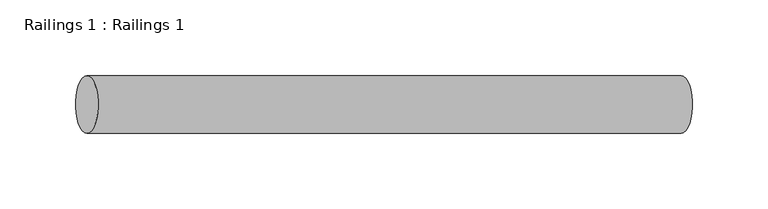
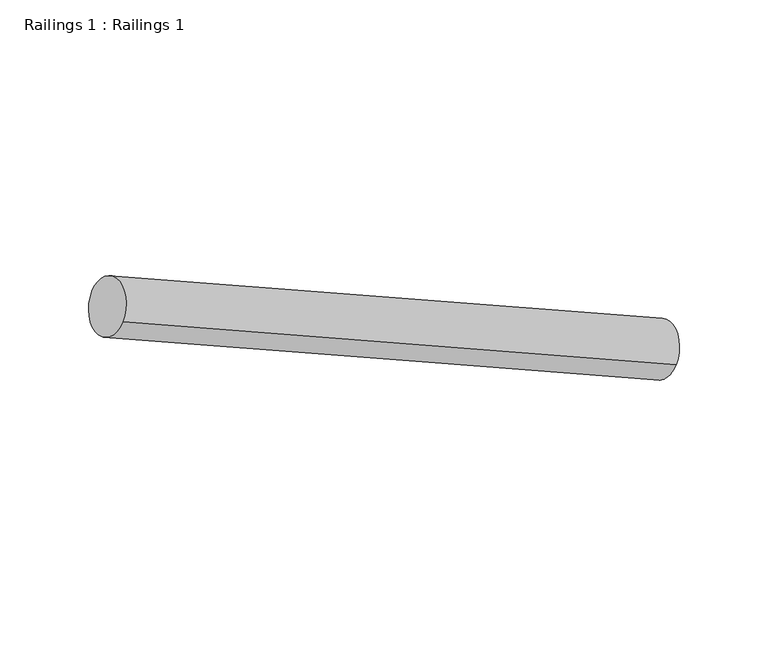
"""IFC4 building model written with IfcOpenShell, lengths in millimetres: railing geometry, Railings 1 : Railings 1."""

from ifc_helpers import new_model, si_unit, point, frame, frame_2d, origin, place, context, project, spatial, circle_curve, trimmed, segment, composite_curve, outline, extrude, source, transform, mapped, element, save


def railings_1_railings_1_71f28f68(model_context):
    return source(origin(), model_context, "Body", "SweptSolid", [
        extrude(outline(composite_curve([segment(trimmed(circle_curve(frame_2d((0.0, -19.05)), 19.05), [point((0.0, -38.1))], [point((0.0, 0.0))], False, "CARTESIAN"), True, "CONTINUOUS"), segment(trimmed(circle_curve(frame_2d((0.0, -19.05)), 19.05), [point((0.0, 0.0))], [point((0.0, -38.1))], False, "CARTESIAN"), True, "CONTINUOUS")], self_intersect=False)), frame((27413.4762341, 3829.6727004, 2323.0746661), z_axis=(-0.9180751215985248, 0.0, 0.39640644684698806), x_axis=(-0.39640644684698806, 0.0, -0.9180751215985248)), (0.0, 0.0, 1.0), 428.2410903),
    ])


if __name__ == "__main__":
    model = new_model("IFC4")
    model_context = context("Model", 3, world=origin())
    ifc_project = project(units=[si_unit("LENGTHUNIT", "METRE", prefix="MILLI")], contexts=[model_context])
    site = spatial("IfcSite", under=ifc_project)
    building = spatial("IfcBuilding", under=site)
    placement = place(None, origin())
    railings_1_railings_1_shape = railings_1_railings_1_71f28f68(model_context)
    element("IfcRailing", 1, ObjectType="Railings 1 : Railings 1", at=placement, inside=building, context=model_context, shape_type="MappedRepresentation", body=[
        mapped(railings_1_railings_1_shape, transform((0.0, 0.0, 0.0), x_axis=(1.0, 0.0, 0.0), y_axis=(0.0, 1.0, 0.0), z_axis=(0.0, 0.0, 1.0))),
    ])
    save(model, "model.ifc")

# Revit data of these elements
# Element 1 (IfcRailing, "Railings 1 : Railings 1")
#   Materials on its faces: "1 1/2\" DIA. HANDRAIL (1 1/2\" MIN. CLEAR FROM WALL)"
# Materials
#   "1 1/2\" DIA. HANDRAIL (1 1/2\" MIN. CLEAR FROM WALL)": class "Unassigned", colour RGB 199 199 199, transparency 0, Cost = 0
